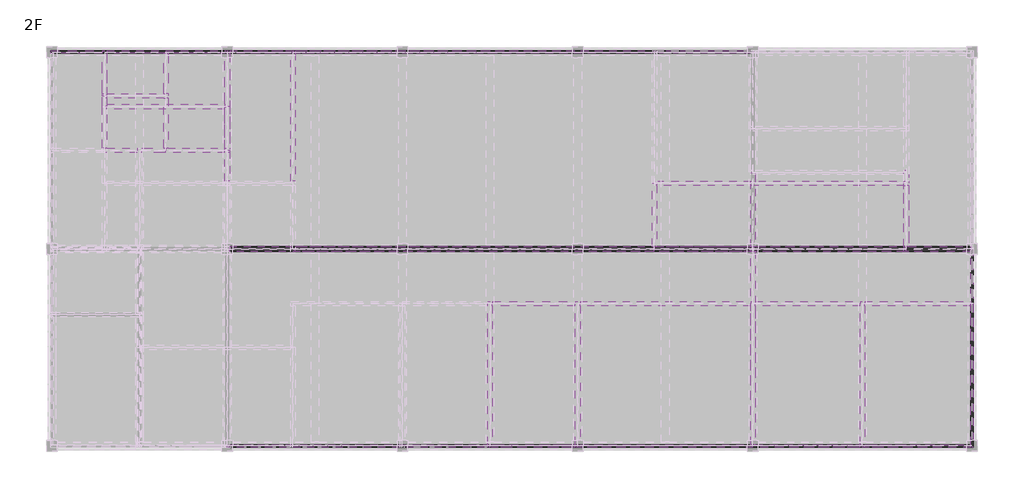
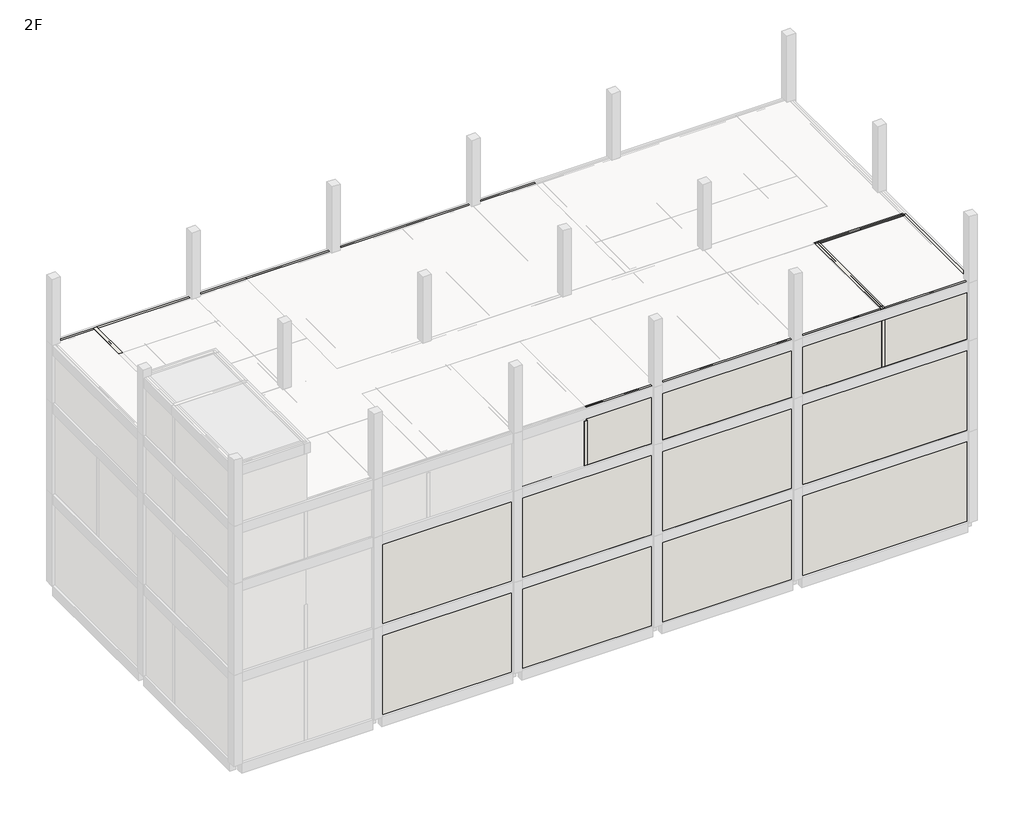
# One storey, part 2 of 7: 54 walls.
"""IFC4 building model written with IfcOpenShell, lengths in millimetres."""

from ifc_helpers import new_model, si_unit, frame, origin, place, context, project, spatial, polyline, outline, extrude, faceted_brep, element, save

model = new_model("IFC4")

# Units and contexts
model_context = context("Model", 3, world=origin())
ifc_project = project(units=[si_unit("LENGTHUNIT", "METRE", prefix="MILLI")], contexts=[model_context])

# Site, building, storey
site = spatial("IfcSite", under=ifc_project)
building = spatial("IfcBuilding", under=site)
storey = spatial("IfcBuildingStorey", under=building, Name="2F", Elevation=3500.0)

# Walls
placement = place(None, origin())
element("IfcWall", 1, ObjectType="WA211_Exterior-Cement Brick-90mm", at=placement, inside=storey, context=model_context, shape_type="Brep", body=[
    faceted_brep([(45402.6521483, 181866.8614395, 3500.0), (45516.6521483, 181866.8614395, 3500.0), (77352.6521483, 181866.8614395, 3500.0), (77352.6521483, 181866.8614395, 9000.0), (45516.6521483, 181866.8614395, 9000.0), (45402.6521483, 181866.8614395, 9000.0), (45402.6521483, 181980.8614395, 3500.0), (45402.6521483, 181980.8614395, 9000.0), (77352.6521483, 181980.8614395, 9000.0), (77352.6521483, 181980.8614395, 3500.0)], [[[0, 1, 2, 3, 4, 5]], [[6, 7, 8, 9]], [[2, 1, 0, 6, 9]], [[5, 4, 3, 8, 7]], [[0, 5, 7, 6]], [[3, 2, 9, 8]]]),
])
element("IfcWall", 2, ObjectType="WA211_Exterior-Cement Brick-90mm", at=placement, inside=storey, context=model_context, shape_type="SweptSolid", body=[
    extrude(outline(polyline([(53566.6521483, 163980.8614395), (87402.6521483, 163980.8614395), (87402.6521483, 163866.8614395), (53566.6521483, 163866.8614395), (53566.6521483, 163980.8614395)])), frame((0.0, 0.0, 3500.0), z_axis=(0.0, 0.0, 1.0), x_axis=(1.0, 0.0, 0.0)), (0.0, 0.0, 1.0), 5500.0),
])
element("IfcWall", 3, ObjectType="WA211_Exterior-Cement Brick-90mm", at=placement, inside=storey, context=model_context, shape_type="Brep", body=[
    faceted_brep([(87402.6521483, 172923.8614395, 3500.0), (87402.6521483, 172816.8614395, 3500.0), (87402.6521483, 163980.8614395, 3500.0), (87402.6521483, 163866.8614395, 3500.0), (87402.6521483, 163866.8614395, 9000.0), (87402.6521483, 163980.8614395, 9000.0), (87402.6521483, 172816.8614395, 9000.0), (87402.6521483, 172923.8614395, 9000.0), (87516.6521483, 172923.8614395, 3500.0), (87516.6521483, 172923.8614395, 9000.0), (87516.6521483, 163866.8614395, 9000.0), (87516.6521483, 163866.8614395, 3500.0)], [[[0, 1, 2, 3, 4, 5, 6, 7]], [[8, 9, 10, 11]], [[3, 2, 1, 0, 8, 11]], [[7, 6, 5, 4, 10, 9]], [[0, 7, 9, 8]], [[4, 3, 11, 10]]]),
])
element("IfcWall", 4, ObjectType="WA211_Exterior-Cement Brick-90mm", at=placement, inside=storey, context=model_context, shape_type="SweptSolid", body=[
    extrude(outline(polyline([(9000.0, 53566.6521483), (9000.0, 77352.6521483), (12400.0, 77352.6521483), (12400.0, 77459.6521483), (14500.0, 77459.6521483), (14500.0, 53459.6521483), (12400.0, 53459.6521483), (12400.0, 53566.6521483), (9000.0, 53566.6521483)])), frame((0.0, 181866.8614395, 0.0), z_axis=(0.0, 1.0, 0.0), x_axis=(0.0, 0.0, 1.0)), (0.0, 0.0, 1.0), 114.0),
])
element("IfcWall", 5, ObjectType="WA211_Exterior-Cement Brick-90mm", at=placement, inside=storey, context=model_context, shape_type="Brep", body=[
    faceted_brep([(77459.6521483, 163980.8614395, 9000.0), (77352.6521483, 163980.8614395, 9000.0), (53566.6521483, 163980.8614395, 9000.0), (53566.6521483, 163980.8614395, 12000.0), (53459.6521483, 163980.8614395, 12000.0), (53459.6521483, 163980.8614395, 14500.0), (77352.6521483, 163980.8614395, 14500.0), (77459.6521483, 163980.8614395, 14500.0), (77459.6521483, 163866.8614395, 9000.0), (77459.6521483, 163866.8614395, 14500.0), (53459.6521483, 163866.8614395, 14500.0), (53459.6521483, 163866.8614395, 12000.0), (53566.6521483, 163866.8614395, 12000.0), (53566.6521483, 163866.8614395, 9000.0)], [[[0, 1, 2, 3, 4, 5, 6, 7]], [[8, 9, 10, 11, 12, 13]], [[2, 1, 0, 8, 13]], [[7, 6, 5, 10, 9]], [[0, 7, 9, 8]], [[5, 4, 11, 10]], [[11, 4, 3, 12]], [[3, 2, 13, 12]]]),
])
element("IfcWall", 6, ObjectType="WA211_Exterior-Cement Brick-90mm", at=placement, inside=storey, context=model_context, shape_type="Brep", body=[
    faceted_brep([(87402.6521483, 163980.8614395, 9000.0), (77566.6521483, 163980.8614395, 9000.0), (77459.6521483, 163980.8614395, 9000.0), (77459.6521483, 163980.8614395, 14500.0), (77566.6521483, 163980.8614395, 14500.0), (87402.6521483, 163980.8614395, 14500.0), (87402.6521483, 163866.8614395, 9000.0), (87402.6521483, 163866.8614395, 14500.0), (77459.6521483, 163866.8614395, 14500.0), (77459.6521483, 163866.8614395, 9000.0)], [[[0, 1, 2, 3, 4, 5]], [[6, 7, 8, 9]], [[2, 1, 0, 6, 9]], [[3, 2, 9, 8]], [[5, 4, 3, 8, 7]], [[0, 5, 7, 6]]]),
])
element("IfcWall", 7, ObjectType="WA211_Exterior-Cement Brick-90mm", at=placement, inside=storey, context=model_context, shape_type="Brep", body=[
    faceted_brep([(87402.6521483, 172923.8614395, 9000.0), (87402.6521483, 172816.8614395, 9000.0), (87402.6521483, 163980.8614395, 9000.0), (87402.6521483, 163866.8614395, 9000.0), (87402.6521483, 163866.8614395, 14500.0), (87402.6521483, 163980.8614395, 14500.0), (87402.6521483, 172816.8614395, 14500.0), (87402.6521483, 172923.8614395, 14500.0), (87516.6521483, 172923.8614395, 9000.0), (87516.6521483, 172923.8614395, 14500.0), (87516.6521483, 163866.8614395, 14500.0), (87516.6521483, 163866.8614395, 9000.0)], [[[0, 1, 2, 3, 4, 5, 6, 7]], [[8, 9, 10, 11]], [[3, 2, 1, 0, 8, 11]], [[7, 6, 5, 4, 10, 9]], [[0, 7, 9, 8]], [[4, 3, 11, 10]]]),
])
element("IfcWall", 8, ObjectType="WA211_Exterior-Cement Brick-90mm", at=placement, inside=storey, context=model_context, shape_type="Brep", body=[
    faceted_brep([(45402.6521483, 181866.8614395, 9000.0), (45516.6521483, 181866.8614395, 9000.0), (47752.6521483, 181866.8614395, 9000.0), (47752.6521483, 181866.8614395, 14500.0), (45516.6521483, 181866.8614395, 14500.0), (45402.6521483, 181866.8614395, 14500.0), (45402.6521483, 181980.8614395, 9000.0), (45402.6521483, 181980.8614395, 14500.0), (47752.6521483, 181980.8614395, 14500.0), (47752.6521483, 181980.8614395, 9000.0)], [[[0, 1, 2, 3, 4, 5]], [[6, 7, 8, 9]], [[2, 1, 0, 6, 9]], [[5, 4, 3, 8, 7]], [[0, 5, 7, 6]], [[3, 2, 9, 8]]]),
])
element("IfcWall", 9, ObjectType="WA211_Exterior-Cement Brick-90mm", at=placement, inside=storey, context=model_context, shape_type="Brep", body=[
    faceted_brep([(50659.6521483, 181866.8614395, 14500.0), (50659.6521483, 181866.8614395, 9000.0), (50766.6521483, 181866.8614395, 9000.0), (53352.6521483, 181866.8614395, 9000.0), (53352.6521483, 181866.8614395, 12400.0), (53459.6521483, 181866.8614395, 12400.0), (53459.6521483, 181866.8614395, 14500.0), (50659.6521483, 181980.8614395, 9000.0), (50659.6521483, 181980.8614395, 14500.0), (53459.6521483, 181980.8614395, 14500.0), (53459.6521483, 181980.8614395, 12400.0), (53352.6521483, 181980.8614395, 12400.0), (53352.6521483, 181980.8614395, 9000.0)], [[[0, 1, 2, 3, 4, 5, 6]], [[7, 8, 9, 10, 11, 12]], [[3, 2, 1, 7, 12]], [[0, 6, 9, 8]], [[6, 5, 10, 9]], [[10, 5, 4, 11]], [[4, 3, 12, 11]], [[0, 8, 7, 1]]]),
])
element("IfcWall", 10, ObjectType="WA211_Exterior-Cement Brick-90mm", at=placement, inside=storey, context=model_context, shape_type="Brep", body=[
    faceted_brep([(47966.6521483, 181866.8614395, 9000.0), (50552.6521483, 181866.8614395, 9000.0), (50659.6521483, 181866.8614395, 9000.0), (50659.6521483, 181866.8614395, 14500.0), (47966.6521483, 181866.8614395, 14500.0), (47966.6521483, 181980.8614395, 9000.0), (47966.6521483, 181980.8614395, 14500.0), (50659.6521483, 181980.8614395, 14500.0), (50659.6521483, 181980.8614395, 9000.0)], [[[0, 1, 2, 3, 4]], [[5, 6, 7, 8]], [[2, 1, 0, 5, 8]], [[4, 3, 7, 6]], [[0, 4, 6, 5]], [[2, 8, 7, 3]]]),
])
element("IfcWall", 11, ObjectType="WA211_Exterior-Cement Brick-90mm", at=placement, inside=storey, context=model_context, shape_type="SweptSolid", body=[
    extrude(outline(polyline([(14500.0, 69352.6521483), (17200.0, 69352.6521483), (17200.0, 69459.6521483), (18000.0, 69459.6521483), (18000.0, 65459.6521483), (17200.0, 65459.6521483), (17200.0, 65566.6521483), (14500.0, 65566.6521483), (14500.0, 69352.6521483)])), frame((0.0, 163866.8614395, 0.0), z_axis=(0.0, 1.0, 0.0), x_axis=(0.0, 0.0, 1.0)), (0.0, 0.0, 1.0), 114.0),
])
element("IfcWall", 12, ObjectType="WA211_Exterior-Cement Brick-90mm", at=placement, inside=storey, context=model_context, shape_type="Brep", body=[
    faceted_brep([(77459.6521483, 163980.8614395, 18000.0), (77459.6521483, 163980.8614395, 14500.0), (77352.6521483, 163980.8614395, 14500.0), (69566.6521483, 163980.8614395, 14500.0), (69566.6521483, 163980.8614395, 17200.0), (69459.6521483, 163980.8614395, 17200.0), (69459.6521483, 163980.8614395, 18000.0), (77459.6521483, 163866.8614395, 14500.0), (77459.6521483, 163866.8614395, 18000.0), (69459.6521483, 163866.8614395, 18000.0), (69459.6521483, 163866.8614395, 17200.0), (69566.6521483, 163866.8614395, 17200.0), (69566.6521483, 163866.8614395, 14500.0)], [[[0, 1, 2, 3, 4, 5, 6]], [[7, 8, 9, 10, 11, 12]], [[3, 2, 1, 7, 12]], [[0, 6, 9, 8]], [[6, 5, 10, 9]], [[10, 5, 4, 11]], [[4, 3, 12, 11]], [[0, 8, 7, 1]]]),
])
element("IfcWall", 13, ObjectType="WA211_Exterior-Cement Brick-90mm", at=placement, inside=storey, context=model_context, shape_type="SweptSolid", body=[
    extrude(outline(polyline([(14500.0, 56566.6521483), (14500.0, 72852.6521483), (17200.0, 72852.6521483), (17200.0, 72959.6521483), (18000.0, 72959.6521483), (18000.0, 56459.6521483), (17200.0, 56459.6521483), (17200.0, 56566.6521483), (14500.0, 56566.6521483)])), frame((0.0, 181866.8614395, 0.0), z_axis=(0.0, 1.0, 0.0), x_axis=(0.0, 0.0, 1.0)), (0.0, 0.0, 1.0), 114.0),
])
element("IfcWall", 14, ObjectType="WA211_Exterior-Cement Brick-90mm", at=placement, inside=storey, context=model_context, shape_type="Brep", body=[
    faceted_brep([(82352.6521483, 163980.8614395, 14500.0), (77566.6521483, 163980.8614395, 14500.0), (77459.6521483, 163980.8614395, 14500.0), (77459.6521483, 163980.8614395, 18000.0), (82352.6521483, 163980.8614395, 18000.0), (82352.6521483, 163866.8614395, 14500.0), (82352.6521483, 163866.8614395, 18000.0), (77459.6521483, 163866.8614395, 18000.0), (77459.6521483, 163866.8614395, 14500.0)], [[[0, 1, 2, 3, 4]], [[5, 6, 7, 8]], [[2, 1, 0, 5, 8]], [[4, 3, 7, 6]], [[2, 8, 7, 3]], [[0, 4, 6, 5]]]),
])
element("IfcWall", 15, ObjectType="WA211_Exterior-Cement Brick-90mm", at=placement, inside=storey, context=model_context, shape_type="SweptSolid", body=[
    extrude(outline(polyline([(82566.6521483, 163980.8614395), (87402.6521483, 163980.8614395), (87402.6521483, 163866.8614395), (82566.6521483, 163866.8614395), (82566.6521483, 163980.8614395)])), frame((0.0, 0.0, 14500.0), z_axis=(0.0, 0.0, 1.0), x_axis=(1.0, 0.0, 0.0)), (0.0, 0.0, 1.0), 3500.0),
])
element("IfcWall", 16, ObjectType="WA211_Exterior-Cement Brick-90mm", at=placement, inside=storey, context=model_context, shape_type="Brep", body=[
    faceted_brep([(87402.6521483, 170423.8614395, 14500.0), (87402.6521483, 170316.8614395, 14500.0), (87402.6521483, 163980.8614395, 14500.0), (87402.6521483, 163866.8614395, 14500.0), (87402.6521483, 163866.8614395, 18000.0), (87402.6521483, 163980.8614395, 18000.0), (87402.6521483, 170316.8614395, 18000.0), (87402.6521483, 170423.8614395, 18000.0), (87516.6521483, 170423.8614395, 14500.0), (87516.6521483, 170423.8614395, 18000.0), (87516.6521483, 163866.8614395, 18000.0), (87516.6521483, 163866.8614395, 14500.0)], [[[0, 1, 2, 3, 4, 5, 6, 7]], [[8, 9, 10, 11]], [[3, 2, 1, 0, 8, 11]], [[7, 6, 5, 4, 10, 9]], [[0, 7, 9, 8]], [[4, 3, 11, 10]]]),
])
element("IfcWall", 17, ObjectType="WA211_Exterior-Cement Brick-90mm", at=placement, inside=storey, context=model_context, shape_type="SweptSolid", body=[
    extrude(outline(polyline([(14500.0, 47966.6521483), (14500.0, 53352.6521483), (17200.0, 53352.6521483), (17200.0, 53459.6521483), (18000.0, 53459.6521483), (18000.0, 47966.6521483), (14500.0, 47966.6521483)])), frame((0.0, 181866.8614395, 0.0), z_axis=(0.0, 1.0, 0.0), x_axis=(0.0, 0.0, 1.0)), (0.0, 0.0, 1.0), 114.0),
])
element("IfcWall", 18, ObjectType="WA211_Exterior-Cement Brick-90mm", at=placement, inside=storey, context=model_context, shape_type="SweptSolid", body=[
    extrude(outline(polyline([(14500.0, 53566.6521483), (14500.0, 56352.6521483), (17200.0, 56352.6521483), (17200.0, 56459.6521483), (18000.0, 56459.6521483), (18000.0, 53459.6521483), (17200.0, 53459.6521483), (17200.0, 53566.6521483), (14500.0, 53566.6521483)])), frame((0.0, 181866.8614395, 0.0), z_axis=(0.0, 1.0, 0.0), x_axis=(0.0, 0.0, 1.0)), (0.0, 0.0, 1.0), 114.0),
])
element("IfcWall", 19, ObjectType="WA211_Exterior-Cement Brick-90mm", at=placement, inside=storey, context=model_context, shape_type="Brep", body=[
    faceted_brep([(45402.6521483, 181866.8614395, 14500.0), (45516.6521483, 181866.8614395, 14500.0), (47752.6521483, 181866.8614395, 14500.0), (47752.6521483, 181866.8614395, 18000.0), (45516.6521483, 181866.8614395, 18000.0), (45402.6521483, 181866.8614395, 18000.0), (45402.6521483, 181980.8614395, 14500.0), (45402.6521483, 181980.8614395, 18000.0), (47752.6521483, 181980.8614395, 18000.0), (47752.6521483, 181980.8614395, 14500.0)], [[[0, 1, 2, 3, 4, 5]], [[6, 7, 8, 9]], [[2, 1, 0, 6, 9]], [[5, 4, 3, 8, 7]], [[3, 2, 9, 8]], [[0, 5, 7, 6]]]),
])
element("IfcWall", 20, ObjectType="WA221_Interior-Cement Block-190mm", at=placement, inside=storey, context=model_context, shape_type="SweptSolid", body=[
    extrude(outline(polyline([(53566.6521483, 173030.8614395), (77352.6521483, 173030.8614395), (77352.6521483, 172816.8614395), (53566.6521483, 172816.8614395), (53566.6521483, 173030.8614395)])), frame((0.0, 0.0, 3500.0), z_axis=(0.0, 0.0, 1.0), x_axis=(1.0, 0.0, 0.0)), (0.0, 0.0, 1.0), 5500.0),
])
element("IfcWall", 21, ObjectType="WA221_Interior-Cement Block-190mm", at=placement, inside=storey, context=model_context, shape_type="Brep", body=[
    faceted_brep([(77566.6521483, 172816.8614395, 3500.0), (87402.6521483, 172816.8614395, 3500.0), (87402.6521483, 172816.8614395, 9000.0), (77566.6521483, 172816.8614395, 9000.0), (77566.6521483, 173030.8614395, 3500.0), (77566.6521483, 173030.8614395, 9000.0), (87402.6521483, 173030.8614395, 9000.0), (87402.6521483, 173030.8614395, 3500.0), (87402.6521483, 172923.8614395, 3500.0), (87402.6521483, 172923.8614395, 9000.0)], [[[0, 1, 2, 3]], [[4, 5, 6, 7]], [[1, 0, 4, 7, 8]], [[3, 2, 9, 6, 5]], [[0, 3, 5, 4]], [[2, 1, 8, 7, 6, 9]]]),
])
element("IfcWall", 22, ObjectType="WA221_Interior-Cement Block-190mm", at=placement, inside=storey, context=model_context, shape_type="Brep", body=[
    faceted_brep([(77459.6521483, 173030.8614395, 9000.0), (77352.6521483, 173030.8614395, 9000.0), (53566.6521483, 173030.8614395, 9000.0), (53566.6521483, 173030.8614395, 12400.0), (77352.6521483, 173030.8614395, 12400.0), (77459.6521483, 173030.8614395, 12400.0), (77459.6521483, 172816.8614395, 9000.0), (77459.6521483, 172816.8614395, 12400.0), (77352.6521483, 172816.8614395, 12400.0), (53566.6521483, 172816.8614395, 12400.0), (53566.6521483, 172816.8614395, 12000.0), (53566.6521483, 172816.8614395, 9000.0), (77352.6521483, 172816.8614395, 9000.0), (53566.6521483, 172923.8614395, 9000.0)], [[[0, 1, 2, 3, 4, 5]], [[6, 7, 8, 9, 10, 11, 12]], [[2, 1, 0, 6, 12, 11, 13]], [[5, 4, 3, 9, 8, 7]], [[0, 5, 7, 6]], [[2, 13, 11, 10, 9, 3]]]),
])
element("IfcWall", 23, ObjectType="WA221_Interior-Cement Block-190mm", at=placement, inside=storey, context=model_context, shape_type="Brep", body=[
    faceted_brep([(77352.6521483, 176316.8614395, 9000.0), (77352.6521483, 173030.8614395, 9000.0), (77352.6521483, 173030.8614395, 12400.0), (77352.6521483, 176423.8614395, 12400.0), (77352.6521483, 176423.8614395, 11700.0), (77352.6521483, 176316.8614395, 11700.0), (77566.6521483, 176316.8614395, 9000.0), (77566.6521483, 176316.8614395, 11700.0), (77566.6521483, 176423.8614395, 11700.0), (77566.6521483, 176423.8614395, 12400.0), (77566.6521483, 173030.8614395, 12400.0), (77566.6521483, 173030.8614395, 9000.0), (77459.6521483, 173030.8614395, 9000.0), (77459.6521483, 173030.8614395, 12400.0)], [[[0, 1, 2, 3, 4, 5]], [[6, 7, 8, 9, 10, 11]], [[1, 0, 6, 11, 12]], [[3, 2, 13, 10, 9]], [[2, 1, 12, 11, 10, 13]], [[4, 3, 9, 8]], [[4, 8, 7, 5]], [[0, 5, 7, 6]]]),
])
element("IfcWall", 24, ObjectType="WA221_Interior-Cement Block-190mm", at=placement, inside=storey, context=model_context, shape_type="Brep", body=[
    faceted_brep([(53566.6521483, 177530.8614395, 9000.0), (53566.6521483, 181866.8614395, 9000.0), (53566.6521483, 181980.8614395, 9000.0), (53566.6521483, 181980.8614395, 12400.0), (53566.6521483, 181866.8614395, 12400.0), (53566.6521483, 177423.8614395, 12400.0), (53566.6521483, 177423.8614395, 11700.0), (53566.6521483, 177530.8614395, 11700.0), (53352.6521483, 177530.8614395, 9000.0), (53352.6521483, 177530.8614395, 11700.0), (53352.6521483, 177423.8614395, 11700.0), (53352.6521483, 177423.8614395, 12400.0), (53352.6521483, 181866.8614395, 12400.0), (53352.6521483, 181980.8614395, 12400.0), (53352.6521483, 181980.8614395, 9000.0), (53352.6521483, 181866.8614395, 9000.0), (53459.6521483, 181980.8614395, 12400.0)], [[[0, 1, 2, 3, 4, 5, 6, 7]], [[8, 9, 10, 11, 12, 13, 14, 15]], [[2, 1, 0, 8, 15, 14]], [[5, 4, 3, 16, 13, 12, 11]], [[3, 2, 14, 13, 16]], [[6, 5, 11, 10]], [[6, 10, 9, 7]], [[0, 7, 9, 8]]]),
])
element("IfcWall", 25, ObjectType="WA221_Interior-Cement Block-190mm", at=placement, inside=storey, context=model_context, shape_type="Brep", body=[
    faceted_brep([(77566.6521483, 163980.8614395, 9000.0), (77566.6521483, 172816.8614395, 9000.0), (77566.6521483, 172816.8614395, 14500.0), (77566.6521483, 163980.8614395, 14500.0), (77352.6521483, 163980.8614395, 9000.0), (77352.6521483, 163980.8614395, 14500.0), (77352.6521483, 172816.8614395, 14500.0), (77352.6521483, 172816.8614395, 12400.0), (77352.6521483, 172816.8614395, 9000.0), (77459.6521483, 163980.8614395, 9000.0), (77459.6521483, 172816.8614395, 9000.0), (77459.6521483, 163980.8614395, 14500.0)], [[[0, 1, 2, 3]], [[4, 5, 6, 7, 8]], [[1, 0, 9, 4, 8, 10]], [[3, 2, 6, 5, 11]], [[1, 10, 8, 7, 6, 2]], [[0, 3, 11, 5, 4, 9]]]),
])
element("IfcWall", 26, ObjectType="WA221_Interior-Cement Block-190mm", at=placement, inside=storey, context=model_context, shape_type="Brep", body=[
    faceted_brep([(77459.6521483, 172816.8614395, 9000.0), (77566.6521483, 172816.8614395, 9000.0), (84459.6521483, 172816.8614395, 9000.0), (84459.6521483, 172816.8614395, 14500.0), (77566.6521483, 172816.8614395, 14500.0), (77352.6521483, 172816.8614395, 14500.0), (77352.6521483, 172816.8614395, 12400.0), (77459.6521483, 172816.8614395, 12400.0), (77459.6521483, 173030.8614395, 9000.0), (77459.6521483, 173030.8614395, 12400.0), (77352.6521483, 173030.8614395, 12400.0), (77352.6521483, 173030.8614395, 14500.0), (84459.6521483, 173030.8614395, 14500.0), (84459.6521483, 173030.8614395, 9000.0), (84352.6521483, 173030.8614395, 9000.0), (77566.6521483, 173030.8614395, 9000.0)], [[[0, 1, 2, 3, 4, 5, 6, 7]], [[8, 9, 10, 11, 12, 13, 14, 15]], [[2, 1, 0, 8, 15, 14, 13]], [[5, 4, 3, 12, 11]], [[0, 7, 9, 8]], [[6, 10, 9, 7]], [[6, 5, 11, 10]], [[2, 13, 12, 3]]]),
])
element("IfcWall", 27, ObjectType="WA221_Interior-Cement Block-190mm", at=placement, inside=storey, context=model_context, shape_type="Brep", body=[
    faceted_brep([(84459.6521483, 172816.8614395, 14500.0), (84459.6521483, 172816.8614395, 9000.0), (87402.6521483, 172816.8614395, 9000.0), (87402.6521483, 172816.8614395, 14500.0), (84459.6521483, 173030.8614395, 9000.0), (84459.6521483, 173030.8614395, 14500.0), (87402.6521483, 173030.8614395, 14500.0), (87402.6521483, 173030.8614395, 9000.0), (84566.6521483, 173030.8614395, 9000.0), (87402.6521483, 172923.8614395, 9000.0), (87402.6521483, 172923.8614395, 14500.0)], [[[0, 1, 2, 3]], [[4, 5, 6, 7, 8]], [[2, 1, 4, 8, 7, 9]], [[0, 3, 10, 6, 5]], [[3, 2, 9, 7, 6, 10]], [[0, 5, 4, 1]]]),
])
element("IfcWall", 28, ObjectType="WA221_Interior-Cement Block-190mm", at=placement, inside=storey, context=model_context, shape_type="Brep", body=[
    faceted_brep([(84352.6521483, 176530.8614395, 9000.0), (84352.6521483, 176316.8614395, 9000.0), (84352.6521483, 173030.8614395, 9000.0), (84352.6521483, 173030.8614395, 11700.0), (84352.6521483, 176316.8614395, 11700.0), (84352.6521483, 176530.8614395, 11700.0), (84566.6521483, 176530.8614395, 9000.0), (84566.6521483, 176530.8614395, 11700.0), (84566.6521483, 173030.8614395, 11700.0), (84566.6521483, 173030.8614395, 9000.0), (84459.6521483, 173030.8614395, 9000.0)], [[[0, 1, 2, 3, 4, 5]], [[6, 7, 8, 9]], [[2, 1, 0, 6, 9, 10]], [[5, 4, 3, 8, 7]], [[0, 5, 7, 6]], [[3, 2, 10, 9, 8]]]),
])
element("IfcWall", 29, ObjectType="WA221_Interior-Cement Block-190mm", at=placement, inside=storey, context=model_context, shape_type="Brep", body=[
    faceted_brep([(47752.6521483, 181980.8614395, 9000.0), (47752.6521483, 181866.8614395, 9000.0), (47752.6521483, 180030.8614395, 9000.0), (47752.6521483, 180030.8614395, 11700.0), (47752.6521483, 179923.8614395, 11700.0), (47752.6521483, 179923.8614395, 14500.0), (47752.6521483, 181866.8614395, 14500.0), (47752.6521483, 181980.8614395, 14500.0), (47966.6521483, 181980.8614395, 9000.0), (47966.6521483, 181980.8614395, 14500.0), (47966.6521483, 181866.8614395, 14500.0), (47966.6521483, 179923.8614395, 14500.0), (47966.6521483, 179923.8614395, 11700.0), (47966.6521483, 180030.8614395, 11700.0), (47966.6521483, 180030.8614395, 9000.0), (47966.6521483, 181866.8614395, 9000.0)], [[[0, 1, 2, 3, 4, 5, 6, 7]], [[8, 9, 10, 11, 12, 13, 14, 15]], [[2, 1, 0, 8, 15, 14]], [[7, 6, 5, 11, 10, 9]], [[0, 7, 9, 8]], [[5, 4, 12, 11]], [[12, 4, 3, 13]], [[3, 2, 14, 13]]]),
])
element("IfcWall", 30, ObjectType="WA221_Interior-Cement Block-190mm", at=placement, inside=storey, context=model_context, shape_type="Brep", body=[
    faceted_brep([(47752.6521483, 179816.8614395, 9000.0), (47752.6521483, 177530.8614395, 9000.0), (47752.6521483, 177530.8614395, 14500.0), (47752.6521483, 179923.8614395, 14500.0), (47752.6521483, 179923.8614395, 11700.0), (47752.6521483, 179816.8614395, 11700.0), (47966.6521483, 179816.8614395, 9000.0), (47966.6521483, 179816.8614395, 11700.0), (47966.6521483, 179923.8614395, 11700.0), (47966.6521483, 179923.8614395, 14500.0), (47966.6521483, 177530.8614395, 14500.0), (47966.6521483, 177530.8614395, 11700.0), (47966.6521483, 177530.8614395, 9000.0), (47859.6521483, 177530.8614395, 9000.0)], [[[0, 1, 2, 3, 4, 5]], [[6, 7, 8, 9, 10, 11, 12]], [[1, 0, 6, 12, 13]], [[3, 2, 10, 9]], [[1, 13, 12, 11, 10, 2]], [[4, 3, 9, 8]], [[4, 8, 7, 5]], [[0, 5, 7, 6]]]),
])
element("IfcWall", 31, ObjectType="WA221_Interior-Cement Block-190mm", at=placement, inside=storey, context=model_context, shape_type="Brep", body=[
    faceted_brep([(49352.6521483, 177530.8614395, 9000.0), (47966.6521483, 177530.8614395, 9000.0), (47859.6521483, 177530.8614395, 9000.0), (47859.6521483, 177530.8614395, 11700.0), (47966.6521483, 177530.8614395, 11700.0), (49352.6521483, 177530.8614395, 11700.0), (49352.6521483, 177316.8614395, 9000.0), (49352.6521483, 177316.8614395, 11700.0), (47966.6521483, 177316.8614395, 11700.0), (47859.6521483, 177316.8614395, 11700.0), (47859.6521483, 177316.8614395, 9000.0)], [[[0, 1, 2, 3, 4, 5]], [[6, 7, 8, 9, 10]], [[2, 1, 0, 6, 10]], [[3, 2, 10, 9]], [[5, 4, 3, 9, 8, 7]], [[0, 5, 7, 6]]]),
])
element("IfcWall", 32, ObjectType="WA221_Interior-Cement Block-190mm", at=placement, inside=storey, context=model_context, shape_type="Brep", body=[
    faceted_brep([(50552.6521483, 181866.8614395, 9000.0), (50552.6521483, 180030.8614395, 9000.0), (50552.6521483, 180030.8614395, 11700.0), (50552.6521483, 181866.8614395, 11700.0), (50766.6521483, 181866.8614395, 9000.0), (50766.6521483, 181866.8614395, 11700.0), (50766.6521483, 180030.8614395, 11700.0), (50766.6521483, 180030.8614395, 9000.0), (50659.6521483, 181866.8614395, 9000.0)], [[[0, 1, 2, 3]], [[4, 5, 6, 7]], [[1, 0, 8, 4, 7]], [[3, 2, 6, 5]], [[0, 3, 5, 4, 8]], [[2, 1, 7, 6]]]),
])
element("IfcWall", 33, ObjectType="WA221_Interior-Cement Block-190mm", at=placement, inside=storey, context=model_context, shape_type="Brep", body=[
    faceted_brep([(50766.6521483, 177530.8614395, 9000.0), (50766.6521483, 179816.8614395, 9000.0), (50766.6521483, 179816.8614395, 11700.0), (50766.6521483, 177530.8614395, 11700.0), (50552.6521483, 177530.8614395, 9000.0), (50552.6521483, 177530.8614395, 11700.0), (50552.6521483, 179816.8614395, 11700.0), (50552.6521483, 179816.8614395, 9000.0), (50659.6521483, 177530.8614395, 9000.0), (50659.6521483, 177530.8614395, 11700.0)], [[[0, 1, 2, 3]], [[4, 5, 6, 7]], [[1, 0, 8, 4, 7]], [[3, 2, 6, 5, 9]], [[0, 3, 9, 5, 4, 8]], [[2, 1, 7, 6]]]),
])
element("IfcWall", 34, ObjectType="WA221_Interior-Cement Block-190mm", at=placement, inside=storey, context=model_context, shape_type="Brep", body=[
    faceted_brep([(50659.6521483, 177316.8614395, 9000.0), (53352.6521483, 177316.8614395, 9000.0), (53566.6521483, 177316.8614395, 9000.0), (53566.6521483, 177316.8614395, 11700.0), (53352.6521483, 177316.8614395, 11700.0), (50659.6521483, 177316.8614395, 11700.0), (50659.6521483, 177530.8614395, 9000.0), (50659.6521483, 177530.8614395, 11700.0), (50766.6521483, 177530.8614395, 11700.0), (53352.6521483, 177530.8614395, 11700.0), (53566.6521483, 177530.8614395, 11700.0), (53566.6521483, 177530.8614395, 9000.0), (53352.6521483, 177530.8614395, 9000.0), (50766.6521483, 177530.8614395, 9000.0), (53566.6521483, 177423.8614395, 11700.0)], [[[0, 1, 2, 3, 4, 5]], [[6, 7, 8, 9, 10, 11, 12, 13]], [[2, 1, 0, 6, 13, 12, 11]], [[5, 4, 3, 14, 10, 9, 8, 7]], [[0, 5, 7, 6]], [[3, 2, 11, 10, 14]]]),
])
element("IfcWall", 35, ObjectType="WA221_Interior-Cement Block-190mm", at=placement, inside=storey, context=model_context, shape_type="Brep", body=[
    faceted_brep([(50766.6521483, 180030.8614395, 9000.0), (50552.6521483, 180030.8614395, 9000.0), (47966.6521483, 180030.8614395, 9000.0), (47752.6521483, 180030.8614395, 9000.0), (47752.6521483, 180030.8614395, 11700.0), (47966.6521483, 180030.8614395, 11700.0), (50552.6521483, 180030.8614395, 11700.0), (50766.6521483, 180030.8614395, 11700.0), (50766.6521483, 179816.8614395, 9000.0), (50766.6521483, 179816.8614395, 11700.0), (50552.6521483, 179816.8614395, 11700.0), (47966.6521483, 179816.8614395, 11700.0), (47752.6521483, 179816.8614395, 11700.0), (47752.6521483, 179816.8614395, 9000.0), (47966.6521483, 179816.8614395, 9000.0), (50552.6521483, 179816.8614395, 9000.0), (47752.6521483, 179923.8614395, 11700.0)], [[[0, 1, 2, 3, 4, 5, 6, 7]], [[8, 9, 10, 11, 12, 13, 14, 15]], [[3, 2, 1, 0, 8, 15, 14, 13]], [[7, 6, 5, 4, 16, 12, 11, 10, 9]], [[0, 7, 9, 8]], [[4, 3, 13, 12, 16]]]),
])
element("IfcWall", 36, ObjectType="WA221_Interior-Cement Block-190mm", at=placement, inside=storey, context=model_context, shape_type="Brep", body=[
    faceted_brep([(50659.6521483, 177530.8614395, 9000.0), (50552.6521483, 177530.8614395, 9000.0), (49566.6521483, 177530.8614395, 9000.0), (49566.6521483, 177530.8614395, 11700.0), (50552.6521483, 177530.8614395, 11700.0), (50659.6521483, 177530.8614395, 11700.0), (50659.6521483, 177316.8614395, 9000.0), (50659.6521483, 177316.8614395, 11700.0), (49566.6521483, 177316.8614395, 11700.0), (49566.6521483, 177316.8614395, 9000.0)], [[[0, 1, 2, 3, 4, 5]], [[6, 7, 8, 9]], [[2, 1, 0, 6, 9]], [[5, 4, 3, 8, 7]], [[0, 5, 7, 6]], [[3, 2, 9, 8]]]),
])
element("IfcWall", 37, ObjectType="WA221_Interior-Cement Block-190mm", at=placement, inside=storey, context=model_context, shape_type="Brep", body=[
    faceted_brep([(65352.6521483, 170530.8614395, 14500.0), (65352.6521483, 170316.8614395, 14500.0), (65352.6521483, 163980.8614395, 14500.0), (65352.6521483, 163866.8614395, 14500.0), (65352.6521483, 163866.8614395, 17200.0), (65352.6521483, 163980.8614395, 17200.0), (65352.6521483, 170316.8614395, 17200.0), (65352.6521483, 170530.8614395, 17200.0), (65566.6521483, 170530.8614395, 14500.0), (65566.6521483, 170530.8614395, 17200.0), (65566.6521483, 170316.8614395, 17200.0), (65566.6521483, 163980.8614395, 17200.0), (65566.6521483, 163866.8614395, 17200.0), (65566.6521483, 163866.8614395, 14500.0), (65566.6521483, 163980.8614395, 14500.0), (65566.6521483, 170316.8614395, 14500.0), (65459.6521483, 163866.8614395, 17200.0)], [[[0, 1, 2, 3, 4, 5, 6, 7]], [[8, 9, 10, 11, 12, 13, 14, 15]], [[3, 2, 1, 0, 8, 15, 14, 13]], [[7, 6, 5, 4, 16, 12, 11, 10, 9]], [[4, 3, 13, 12, 16]], [[0, 7, 9, 8]]]),
])
element("IfcWall", 38, ObjectType="WA221_Interior-Cement Block-190mm", at=placement, inside=storey, context=model_context, shape_type="Brep", body=[
    faceted_brep([(69566.6521483, 163866.8614395, 14500.0), (69566.6521483, 163980.8614395, 14500.0), (69566.6521483, 170316.8614395, 14500.0), (69566.6521483, 170530.8614395, 14500.0), (69566.6521483, 170530.8614395, 17200.0), (69566.6521483, 170316.8614395, 17200.0), (69566.6521483, 163980.8614395, 17200.0), (69566.6521483, 163866.8614395, 17200.0), (69352.6521483, 163866.8614395, 14500.0), (69352.6521483, 163866.8614395, 17200.0), (69352.6521483, 163980.8614395, 17200.0), (69352.6521483, 170316.8614395, 17200.0), (69352.6521483, 170530.8614395, 17200.0), (69352.6521483, 170530.8614395, 14500.0), (69352.6521483, 170316.8614395, 14500.0), (69352.6521483, 163980.8614395, 14500.0), (69459.6521483, 163866.8614395, 17200.0)], [[[0, 1, 2, 3, 4, 5, 6, 7]], [[8, 9, 10, 11, 12, 13, 14, 15]], [[3, 2, 1, 0, 8, 15, 14, 13]], [[7, 6, 5, 4, 12, 11, 10, 9, 16]], [[4, 3, 13, 12]], [[0, 7, 16, 9, 8]]]),
])
element("IfcWall", 39, ObjectType="WA221_Interior-Cement Block-190mm", at=placement, inside=storey, context=model_context, shape_type="SweptSolid", body=[
    extrude(outline(polyline([(65566.6521483, 170530.8614395), (69352.6521483, 170530.8614395), (69352.6521483, 170316.8614395), (65566.6521483, 170316.8614395), (65566.6521483, 170530.8614395)])), frame((0.0, 0.0, 14500.0), z_axis=(0.0, 0.0, 1.0), x_axis=(1.0, 0.0, 0.0)), (0.0, 0.0, 1.0), 2700.0),
])
element("IfcWall", 40, ObjectType="WA221_Interior-Cement Block-190mm", at=placement, inside=storey, context=model_context, shape_type="Brep", body=[
    faceted_brep([(84566.6521483, 176030.8614395, 14500.0), (84352.6521483, 176030.8614395, 14500.0), (73066.6521483, 176030.8614395, 14500.0), (73066.6521483, 176030.8614395, 17200.0), (84352.6521483, 176030.8614395, 17200.0), (84566.6521483, 176030.8614395, 17200.0), (84566.6521483, 175816.8614395, 14500.0), (84566.6521483, 175816.8614395, 17200.0), (84352.6521483, 175816.8614395, 17200.0), (73066.6521483, 175816.8614395, 17200.0), (73066.6521483, 175816.8614395, 14500.0), (84352.6521483, 175816.8614395, 14500.0), (73066.6521483, 175923.8614395, 14500.0), (73066.6521483, 175923.8614395, 17200.0)], [[[0, 1, 2, 3, 4, 5]], [[6, 7, 8, 9, 10, 11]], [[2, 1, 0, 6, 11, 10, 12]], [[5, 4, 3, 13, 9, 8, 7]], [[0, 5, 7, 6]], [[3, 2, 12, 10, 9, 13]]]),
])
element("IfcWall", 41, ObjectType="WA221_Interior-Cement Block-190mm", at=placement, inside=storey, context=model_context, shape_type="Brep", body=[
    faceted_brep([(77352.6521483, 170530.8614395, 14500.0), (77352.6521483, 170316.8614395, 14500.0), (77352.6521483, 163980.8614395, 14500.0), (77352.6521483, 163980.8614395, 17200.0), (77352.6521483, 170316.8614395, 17200.0), (77352.6521483, 170530.8614395, 17200.0), (77566.6521483, 170530.8614395, 14500.0), (77566.6521483, 170530.8614395, 17200.0), (77566.6521483, 170316.8614395, 17200.0), (77566.6521483, 163980.8614395, 17200.0), (77566.6521483, 163980.8614395, 14500.0), (77566.6521483, 170316.8614395, 14500.0), (77459.6521483, 163980.8614395, 14500.0)], [[[0, 1, 2, 3, 4, 5]], [[6, 7, 8, 9, 10, 11]], [[2, 1, 0, 6, 11, 10, 12]], [[5, 4, 3, 9, 8, 7]], [[0, 5, 7, 6]], [[3, 2, 12, 10, 9]]]),
])
element("IfcWall", 42, ObjectType="WA221_Interior-Cement Block-190mm", at=placement, inside=storey, context=model_context, shape_type="SweptSolid", body=[
    extrude(outline(polyline([(77352.6521483, 170316.8614395), (69566.6521483, 170316.8614395), (69566.6521483, 170530.8614395), (77352.6521483, 170530.8614395), (77352.6521483, 170316.8614395)])), frame((0.0, 0.0, 14500.0), z_axis=(0.0, 0.0, 1.0), x_axis=(1.0, 0.0, 0.0)), (0.0, 0.0, 1.0), 2700.0),
])
element("IfcWall", 43, ObjectType="WA221_Interior-Cement Block-190mm", at=placement, inside=storey, context=model_context, shape_type="Brep", body=[
    faceted_brep([(73066.6521483, 173030.8614395, 14500.0), (73066.6521483, 175816.8614395, 14500.0), (73066.6521483, 175923.8614395, 14500.0), (73066.6521483, 175923.8614395, 17200.0), (73066.6521483, 175816.8614395, 17200.0), (73066.6521483, 173030.8614395, 17200.0), (72852.6521483, 173030.8614395, 14500.0), (72852.6521483, 173030.8614395, 17200.0), (72852.6521483, 175923.8614395, 17200.0), (72852.6521483, 175923.8614395, 14500.0), (72959.6521483, 173030.8614395, 14500.0), (72959.6521483, 173030.8614395, 17200.0)], [[[0, 1, 2, 3, 4, 5]], [[6, 7, 8, 9]], [[2, 1, 0, 10, 6, 9]], [[3, 2, 9, 8]], [[5, 4, 3, 8, 7, 11]], [[0, 5, 11, 7, 6, 10]]]),
])
element("IfcWall", 44, ObjectType="WA221_Interior-Cement Block-190mm", at=placement, inside=storey, context=model_context, shape_type="Brep", body=[
    faceted_brep([(56352.6521483, 181980.8614395, 14500.0), (56352.6521483, 181866.8614395, 14500.0), (56352.6521483, 176030.8614395, 14500.0), (56352.6521483, 176030.8614395, 17200.0), (56352.6521483, 181866.8614395, 17200.0), (56352.6521483, 181980.8614395, 17200.0), (56566.6521483, 181980.8614395, 14500.0), (56566.6521483, 181980.8614395, 17200.0), (56566.6521483, 181866.8614395, 17200.0), (56566.6521483, 176030.8614395, 17200.0), (56566.6521483, 176030.8614395, 14500.0), (56566.6521483, 181866.8614395, 14500.0), (56459.6521483, 181980.8614395, 17200.0)], [[[0, 1, 2, 3, 4, 5]], [[6, 7, 8, 9, 10, 11]], [[2, 1, 0, 6, 11, 10]], [[5, 4, 3, 9, 8, 7, 12]], [[0, 5, 12, 7, 6]], [[3, 2, 10, 9]]]),
])
element("IfcWall", 45, ObjectType="WA221_Interior-Cement Block-190mm", at=placement, inside=storey, context=model_context, shape_type="Brep", body=[
    faceted_brep([(72959.6521483, 173030.8614395, 14500.0), (72852.6521483, 173030.8614395, 14500.0), (56566.6521483, 173030.8614395, 14500.0), (56566.6521483, 173030.8614395, 17200.0), (72852.6521483, 173030.8614395, 17200.0), (72959.6521483, 173030.8614395, 17200.0), (72959.6521483, 172816.8614395, 14500.0), (72959.6521483, 172816.8614395, 17200.0), (56566.6521483, 172816.8614395, 17200.0), (56566.6521483, 172816.8614395, 14500.0)], [[[0, 1, 2, 3, 4, 5]], [[6, 7, 8, 9]], [[2, 1, 0, 6, 9]], [[5, 4, 3, 8, 7]], [[0, 5, 7, 6]], [[3, 2, 9, 8]]]),
])
element("IfcWall", 46, ObjectType="WA221_Interior-Cement Block-190mm", at=placement, inside=storey, context=model_context, shape_type="Brep", body=[
    faceted_brep([(82566.6521483, 163866.8614395, 14500.0), (82566.6521483, 163980.8614395, 14500.0), (82566.6521483, 170316.8614395, 14500.0), (82566.6521483, 170530.8614395, 14500.0), (82566.6521483, 170530.8614395, 18000.0), (82566.6521483, 170316.8614395, 18000.0), (82566.6521483, 163980.8614395, 18000.0), (82566.6521483, 163866.8614395, 18000.0), (82352.6521483, 163866.8614395, 14500.0), (82352.6521483, 163866.8614395, 18000.0), (82352.6521483, 163980.8614395, 18000.0), (82352.6521483, 170530.8614395, 18000.0), (82352.6521483, 170530.8614395, 17200.0), (82352.6521483, 170530.8614395, 14500.0), (82352.6521483, 170316.8614395, 14500.0), (82352.6521483, 163980.8614395, 14500.0)], [[[0, 1, 2, 3, 4, 5, 6, 7]], [[8, 9, 10, 11, 12, 13, 14, 15]], [[3, 2, 1, 0, 8, 15, 14, 13]], [[7, 6, 5, 4, 11, 10, 9]], [[3, 13, 12, 11, 4]], [[0, 7, 9, 8]]]),
])
element("IfcWall", 47, ObjectType="WA221_Interior-Cement Block-190mm", at=placement, inside=storey, context=model_context, shape_type="SweptSolid", body=[
    extrude(outline(polyline([(82352.6521483, 170316.8614395), (77566.6521483, 170316.8614395), (77566.6521483, 170530.8614395), (82352.6521483, 170530.8614395), (82352.6521483, 170316.8614395)])), frame((0.0, 0.0, 14500.0), z_axis=(0.0, 0.0, 1.0), x_axis=(1.0, 0.0, 0.0)), (0.0, 0.0, 1.0), 2700.0),
])
element("IfcWall", 48, ObjectType="WA221_Interior-Cement Block-190mm", at=placement, inside=storey, context=model_context, shape_type="Brep", body=[
    faceted_brep([(82566.6521483, 170316.8614395, 14500.0), (87402.6521483, 170316.8614395, 14500.0), (87402.6521483, 170316.8614395, 18000.0), (82566.6521483, 170316.8614395, 18000.0), (82566.6521483, 170530.8614395, 14500.0), (82566.6521483, 170530.8614395, 18000.0), (87402.6521483, 170530.8614395, 18000.0), (87402.6521483, 170530.8614395, 14500.0), (87402.6521483, 170423.8614395, 14500.0), (87402.6521483, 170423.8614395, 18000.0)], [[[0, 1, 2, 3]], [[4, 5, 6, 7]], [[1, 0, 4, 7, 8]], [[3, 2, 9, 6, 5]], [[0, 3, 5, 4]], [[2, 1, 8, 7, 6, 9]]]),
])
element("IfcWall", 49, ObjectType="WA221_Interior-Cement Block-190mm", at=placement, inside=storey, context=model_context, shape_type="Brep", body=[
    faceted_brep([(84352.6521483, 173030.8614395, 14500.0), (73066.6521483, 173030.8614395, 14500.0), (72959.6521483, 173030.8614395, 14500.0), (72959.6521483, 173030.8614395, 17200.0), (73066.6521483, 173030.8614395, 17200.0), (84352.6521483, 173030.8614395, 17200.0), (84352.6521483, 172816.8614395, 14500.0), (84352.6521483, 172816.8614395, 17200.0), (72959.6521483, 172816.8614395, 17200.0), (72959.6521483, 172816.8614395, 14500.0)], [[[0, 1, 2, 3, 4, 5]], [[6, 7, 8, 9]], [[2, 1, 0, 6, 9]], [[3, 2, 9, 8]], [[5, 4, 3, 8, 7]], [[0, 5, 7, 6]]]),
])
element("IfcWall", 50, ObjectType="WA221_Interior-Cement Block-190mm", at=placement, inside=storey, context=model_context, shape_type="Brep", body=[
    faceted_brep([(84352.6521483, 175816.8614395, 14500.0), (84352.6521483, 173030.8614395, 14500.0), (84352.6521483, 172816.8614395, 14500.0), (84352.6521483, 172816.8614395, 17200.0), (84352.6521483, 173030.8614395, 17200.0), (84352.6521483, 175816.8614395, 17200.0), (84566.6521483, 175816.8614395, 14500.0), (84566.6521483, 175816.8614395, 17200.0), (84566.6521483, 172816.8614395, 17200.0), (84566.6521483, 172816.8614395, 14500.0)], [[[0, 1, 2, 3, 4, 5]], [[6, 7, 8, 9]], [[2, 1, 0, 6, 9]], [[5, 4, 3, 8, 7]], [[0, 5, 7, 6]], [[3, 2, 9, 8]]]),
])
element("IfcWall", 51, ObjectType="WA221_Interior-Cement Block-190mm", at=placement, inside=storey, context=model_context, shape_type="Brep", body=[
    faceted_brep([(53352.6521483, 179530.8614395, 14500.0), (47966.6521483, 179530.8614395, 14500.0), (47966.6521483, 179530.8614395, 17200.0), (53352.6521483, 179530.8614395, 17200.0), (53352.6521483, 179316.8614395, 14500.0), (53352.6521483, 179316.8614395, 17200.0), (47966.6521483, 179316.8614395, 17200.0), (47966.6521483, 179316.8614395, 14500.0), (53352.6521483, 179423.8614395, 14500.0), (47966.6521483, 179423.8614395, 14500.0), (53352.6521483, 179423.8614395, 17200.0)], [[[0, 1, 2, 3]], [[4, 5, 6, 7]], [[1, 0, 8, 4, 7, 9]], [[3, 2, 6, 5, 10]], [[0, 3, 10, 5, 4, 8]], [[2, 1, 9, 7, 6]]]),
])
element("IfcWall", 52, ObjectType="WA221_Interior-Cement Block-190mm", at=placement, inside=storey, context=model_context, shape_type="Brep", body=[
    faceted_brep([(53352.6521483, 179423.8614395, 14500.0), (53352.6521483, 179316.8614395, 14500.0), (53352.6521483, 176030.8614395, 14500.0), (53352.6521483, 176030.8614395, 17200.0), (53352.6521483, 179316.8614395, 17200.0), (53352.6521483, 179423.8614395, 17200.0), (53566.6521483, 179423.8614395, 14500.0), (53566.6521483, 179423.8614395, 17200.0), (53566.6521483, 176030.8614395, 17200.0), (53566.6521483, 176030.8614395, 14500.0), (53459.6521483, 176030.8614395, 14500.0), (53459.6521483, 176030.8614395, 17200.0)], [[[0, 1, 2, 3, 4, 5]], [[6, 7, 8, 9]], [[2, 1, 0, 6, 9, 10]], [[5, 4, 3, 11, 8, 7]], [[0, 5, 7, 6]], [[3, 2, 10, 9, 8, 11]]]),
])
element("IfcWall", 53, ObjectType="WA221_Interior-Cement Block-190mm", at=placement, inside=storey, context=model_context, shape_type="Brep", body=[
    faceted_brep([(53352.6521483, 181980.8614395, 14500.0), (53352.6521483, 181866.8614395, 14500.0), (53352.6521483, 179530.8614395, 14500.0), (53352.6521483, 179423.8614395, 14500.0), (53352.6521483, 179423.8614395, 17200.0), (53352.6521483, 179530.8614395, 17200.0), (53352.6521483, 181866.8614395, 17200.0), (53352.6521483, 181980.8614395, 17200.0), (53566.6521483, 181980.8614395, 14500.0), (53566.6521483, 181980.8614395, 17200.0), (53566.6521483, 181866.8614395, 17200.0), (53566.6521483, 179423.8614395, 17200.0), (53566.6521483, 179423.8614395, 14500.0), (53566.6521483, 181866.8614395, 14500.0), (53459.6521483, 181980.8614395, 17200.0)], [[[0, 1, 2, 3, 4, 5, 6, 7]], [[8, 9, 10, 11, 12, 13]], [[3, 2, 1, 0, 8, 13, 12]], [[4, 3, 12, 11]], [[7, 6, 5, 4, 11, 10, 9, 14]], [[0, 7, 14, 9, 8]]]),
])
element("IfcWall", 54, ObjectType="WA221_Interior-Cement Block-190mm", at=placement, inside=storey, context=model_context, shape_type="Brep", body=[
    faceted_brep([(47752.6521483, 181980.8614395, 14500.0), (47752.6521483, 181866.8614395, 14500.0), (47752.6521483, 179423.8614395, 14500.0), (47752.6521483, 179423.8614395, 18000.0), (47752.6521483, 181866.8614395, 18000.0), (47752.6521483, 181980.8614395, 18000.0), (47966.6521483, 181980.8614395, 14500.0), (47966.6521483, 181980.8614395, 18000.0), (47966.6521483, 181866.8614395, 18000.0), (47966.6521483, 179423.8614395, 18000.0), (47966.6521483, 179423.8614395, 14500.0), (47966.6521483, 179530.8614395, 14500.0), (47966.6521483, 181866.8614395, 14500.0)], [[[0, 1, 2, 3, 4, 5]], [[6, 7, 8, 9, 10, 11, 12]], [[2, 1, 0, 6, 12, 11, 10]], [[5, 4, 3, 9, 8, 7]], [[2, 10, 9, 3]], [[0, 5, 7, 6]]]),
])

save(model, "model.ifc")

# Revit data of these elements
# Type "WA211_Exterior-Cement Brick-90mm"
#   Type Comments = ""
#   Layers, outside or top first: 0 mm "A04AL081-00001_Skirt_Acrylic Emulsion Paint" (function 100); 0 mm "A04AL077-00001_Ext Wall Painting_Acrylic Emulsion Paint" (function 100); 12 mm "A04AS164-00001_Plastering_Ext" (function 4); 90 mm "A04AK073-00001_Concrete Brick_0.5B" (function 1); 12 mm "A04AS164-00002_Plastering_Int" (function 5); 0 mm "A04AL078-00002_Int Wall Painting_Water Emulsion Paint" (function 100); 0 mm "A04AL081-00001_Skirt_Acrylic Emulsion Paint" (function 100)
# Type "WA221_Interior-Cement Block-190mm"
#   Type Comments = ""
#   Layers, outside or top first: 0 mm "A04AL081-00001_Skirt_Acrylic Emulsion Paint" (function 100); 0 mm "A04AL078-00002_Int Wall Painting_Water Emulsion Paint" (function 100); 12 mm "A04AS164-00002_Plastering_Int" (function 2); 190 mm "A04AK069-00002_Reinforced Concrete Block_THK 100-200mm" (function 1); 12 mm "A04AS164-00002_Plastering_Int" (function 2); 0 mm "A04AL078-00002_Int Wall Painting_Water Emulsion Paint" (function 100); 0 mm "A04AL081-00001_Skirt_Acrylic Emulsion Paint" (function 100)
# Elements 1, 3 (IfcWall, "WA211_Exterior-Cement Brick-90mm")
#   Top Offset = 0 mm
#   Base Offset = 0 mm
#   Unconnected Height = 5500 mm
#   wall height = 5500 mm
#   Phase Created = New Construction
#   Base Constraint = 2F
#   Materials on its faces: "Default Wall", "A04AS164-00001_Plastering_Ext", "A04AS164-00002_Plastering_Int"
# Element 2 (IfcWall, "WA211_Exterior-Cement Brick-90mm")
#   Top Offset = 0 mm
#   Base Offset = 0 mm
#   Unconnected Height = 5500 mm
#   wall height = 5500 mm
#   Phase Created = New Construction
#   Base Constraint = 2F
#   Materials on its faces: "Default Wall", "A04AS164-00002_Plastering_Int", "A04AS164-00001_Plastering_Ext"
# Elements 4, 5, 6, 9, 10 (IfcWall, "WA211_Exterior-Cement Brick-90mm")
#   Top Offset = 0 mm
#   Base Offset = 0 mm
#   Unconnected Height = 5500 mm
#   wall height = 5500 mm
#   Phase Created = New Construction
#   Base Constraint = 3F
#   Materials on its faces: "Default Wall", "A04AS164-00002_Plastering_Int", "A04AS164-00001_Plastering_Ext"
# Elements 7, 8 (IfcWall, "WA211_Exterior-Cement Brick-90mm")
#   Top Offset = 0 mm
#   Base Offset = 0 mm
#   Unconnected Height = 5500 mm
#   wall height = 5500 mm
#   Phase Created = New Construction
#   Base Constraint = 3F
#   Materials on its faces: "Default Wall", "A04AS164-00001_Plastering_Ext", "A04AS164-00002_Plastering_Int"
# Elements 11, 12, 13, 14, 15, 17, 18 (IfcWall, "WA211_Exterior-Cement Brick-90mm")
#   Top Offset = 0 mm
#   Base Offset = 0 mm
#   Unconnected Height = 3500 mm
#   wall height = 3500 mm
#   Phase Created = New Construction
#   Base Constraint = 4F
#   Materials on its faces: "Default Wall", "A04AS164-00002_Plastering_Int", "A04AS164-00001_Plastering_Ext"
# Elements 16, 19 (IfcWall, "WA211_Exterior-Cement Brick-90mm")
#   Top Offset = 0 mm
#   Base Offset = 0 mm
#   Unconnected Height = 3500 mm
#   wall height = 3500 mm
#   Phase Created = New Construction
#   Base Constraint = 4F
#   Materials on its faces: "Default Wall", "A04AS164-00001_Plastering_Ext", "A04AS164-00002_Plastering_Int"
# Elements 20, 21 (IfcWall, "WA221_Interior-Cement Block-190mm")
#   Top Offset = 0 mm
#   Base Offset = 0 mm
#   Unconnected Height = 5500 mm
#   wall height = 5500 mm
#   Phase Created = New Construction
#   Base Constraint = 2F
#   Materials on its faces: "Default Wall", "A04AS164-00002_Plastering_Int"
# Elements 22, 23 (IfcWall, "WA221_Interior-Cement Block-190mm")
#   Top Offset = 0 mm
#   Base Offset = 0 mm
#   Unconnected Height = 3400 mm
#   wall height = 3400 mm
#   Phase Created = New Construction
#   Base Constraint = 3F
#   Materials on its faces: "Default Wall", "A04AS164-00002_Plastering_Int"
# Element 24 (IfcWall, "WA221_Interior-Cement Block-190mm")
#   Top Offset = 0 mm
#   Base Offset = 0 mm
#   Unconnected Height = 3400 mm
#   wall height = 3400 mm
#   Phase Created = New Construction
#   Base Constraint = 3F
#   Materials on its faces: "Default Wall", "A04AS164-00002_Plastering_Int", "A04AS164-00001_Plastering_Ext"
# Elements 25, 26, 27, 30 (IfcWall, "WA221_Interior-Cement Block-190mm")
#   Top Offset = 0 mm
#   Base Offset = 0 mm
#   Unconnected Height = 5500 mm
#   wall height = 5500 mm
#   Phase Created = New Construction
#   Base Constraint = 3F
#   Materials on its faces: "Default Wall", "A04AS164-00002_Plastering_Int"
# Elements 28, 34, 35 (IfcWall, "WA221_Interior-Cement Block-190mm")
#   Top Offset = 0 mm
#   Base Offset = 0 mm
#   Unconnected Height = 2700 mm
#   wall height = 2700 mm
#   Phase Created = New Construction
#   Base Constraint = 3F
#   Materials on its faces: "A04AS164-00002_Plastering_Int", "Default Wall"
# Element 29 (IfcWall, "WA221_Interior-Cement Block-190mm")
#   Top Offset = 0 mm
#   Base Offset = 0 mm
#   Unconnected Height = 5500 mm
#   wall height = 5500 mm
#   Phase Created = New Construction
#   Base Constraint = 3F
#   Materials on its faces: "Default Wall", "A04AS164-00002_Plastering_Int", "A04AS164-00001_Plastering_Ext"
# Elements 31, 32, 33, 36 (IfcWall, "WA221_Interior-Cement Block-190mm")
#   Top Offset = 0 mm
#   Base Offset = 0 mm
#   Unconnected Height = 2700 mm
#   wall height = 2700 mm
#   Phase Created = New Construction
#   Base Constraint = 3F
#   Materials on its faces: "Default Wall", "A04AS164-00002_Plastering_Int"
# Elements 37, 38 (IfcWall, "WA221_Interior-Cement Block-190mm")
#   Top Offset = 0 mm
#   Base Offset = 0 mm
#   Unconnected Height = 2700 mm
#   wall height = 2700 mm
#   Phase Created = New Construction
#   Base Constraint = 4F
#   Materials on its faces: "A04AS164-00002_Plastering_Int", "Default Wall", "A04AS164-00001_Plastering_Ext"
# Elements 39, 42, 43, 45, 47, 49, 51, 52 (IfcWall, "WA221_Interior-Cement Block-190mm")
#   Top Offset = 0 mm
#   Base Offset = 0 mm
#   Unconnected Height = 2700 mm
#   wall height = 2700 mm
#   Phase Created = New Construction
#   Base Constraint = 4F
#   Materials on its faces: "Default Wall", "A04AS164-00002_Plastering_Int"
# Elements 40, 41, 50 (IfcWall, "WA221_Interior-Cement Block-190mm")
#   Top Offset = 0 mm
#   Base Offset = 0 mm
#   Unconnected Height = 2700 mm
#   wall height = 2700 mm
#   Phase Created = New Construction
#   Base Constraint = 4F
#   Materials on its faces: "A04AS164-00002_Plastering_Int", "Default Wall"
# Elements 44, 53 (IfcWall, "WA221_Interior-Cement Block-190mm")
#   Top Offset = 0 mm
#   Base Offset = 0 mm
#   Unconnected Height = 2700 mm
#   wall height = 2700 mm
#   Phase Created = New Construction
#   Base Constraint = 4F
#   Materials on its faces: "Default Wall", "A04AS164-00002_Plastering_Int", "A04AS164-00001_Plastering_Ext"
# Element 46 (IfcWall, "WA221_Interior-Cement Block-190mm")
#   Top Offset = 0 mm
#   Base Offset = 0 mm
#   Unconnected Height = 3500 mm
#   wall height = 3500 mm
#   Phase Created = New Construction
#   Base Constraint = 4F
#   Materials on its faces: "A04AS164-00002_Plastering_Int", "Default Wall", "A04AS164-00001_Plastering_Ext"
# Element 48 (IfcWall, "WA221_Interior-Cement Block-190mm")
#   Top Offset = 0 mm
#   Base Offset = 0 mm
#   Unconnected Height = 3500 mm
#   wall height = 3500 mm
#   Phase Created = New Construction
#   Base Constraint = 4F
#   Materials on its faces: "Default Wall", "A04AS164-00002_Plastering_Int"
# Element 54 (IfcWall, "WA221_Interior-Cement Block-190mm")
#   Top Offset = 0 mm
#   Base Offset = 0 mm
#   Unconnected Height = 3500 mm
#   wall height = 3500 mm
#   Phase Created = New Construction
#   Base Constraint = 4F
#   Materials on its faces: "Default Wall", "A04AS164-00002_Plastering_Int", "A04AS164-00001_Plastering_Ext"
# Materials
#   "A04AL081-00001_Skirt_Acrylic Emulsion Paint": class "Finish", colour RGB 128 128 64, transparency 0, Description = "Plastic", W00) Work Master Code = "A04AL081-00001", W01) Work Master_Lv1 = "Finishing Work", W02) Work Master_Lv2 = "Painting Work", W03) Work Master_Spec.1 = "Skirt Painting", W04) Work Master_Spec.2 = "Acrylic Emulsion Paint", W05) Work Master_Spec.3 = "100mm≤H<150mm", Cost = 0
#   "A04AL077-00001_Ext Wall Painting_Acrylic Emulsion Paint": class "Finish", colour RGB 128 128 64, transparency 0, Description = "Plastic", W00) Work Master Code = "A04AL077-00001", W01) Work Master_Lv1 = "Finishing Work", W02) Work Master_Lv2 = "Painting Work", W03) Work Master_Spec.1 = "External Wall Painting", W04) Work Master_Spec.2 = "Acrylic Emulsion Paint", Cost = 0
#   "A04AS164-00001_Plastering_Ext": class "Concrete", colour RGB 183 186 184, transparency 0, W00) Work Master Code = "A04AS164-00001", W01) Work Master_Lv1 = "Finishing Work", W02) Work Master_Lv2 = "Plastering Work", W03) Work Master_Spec.1 = "Plastering", W04) Work Master_Spec.2 = "for External Masonry Wall", Cost = 0
#   "A04AK073-00001_Concrete Brick_0.5B": class "Concrete", colour RGB 180 180 180, transparency 0, Description = "Conc. Block", W00) Work Master Code = "A04AK073-00001", W01) Work Master_Lv1 = "Finishing Work", W02) Work Master_Lv2 = "Masonry Work", W03) Work Master_Spec.1 = "Concrete Brick", W04) Work Master_Spec.2 = "[0.5B] w/ All Reinf.(Lath, Steel Tie, Anchor Bar, Mortar, ETC.), Filler, Sealant, Lintel/Sill for Opening, ETC.", Cost = 0
#   "A04AS164-00002_Plastering_Int": class "Concrete", colour RGB 183 186 184, transparency 0, Description = "LATEX PAINT ON THK.15 CEMENT PLASTER", W00) Work Master Code = "A04AS164-00002", W01) Work Master_Lv1 = "Finishing Work", W02) Work Master_Lv2 = "Plastering Work", W03) Work Master_Spec.1 = "Plastering", W04) Work Master_Spec.2 = "for Internal Masonry Wall", Cost = 0
#   "A04AL078-00002_Int Wall Painting_Water Emulsion Paint": class "Finish", colour RGB 128 128 64, transparency 0, Description = "Plastic", W00) Work Master Code = "A04AL078-00002", W01) Work Master_Lv1 = "Finishing Work", W02) Work Master_Lv2 = "Painting Work", W03) Work Master_Spec.1 = "Internal Wall Painting", W04) Work Master_Spec.2 = "Water Emulsion Paint", Cost = 0
#   "A04AK069-00002_Reinforced Concrete Block_THK 100-200mm": class "Concrete", colour RGB 180 180 180, transparency 0, Description = "Conc. Block", W00) Work Master Code = "A04AK069-00002", W01) Work Master_Lv1 = "Finishing Work", W02) Work Master_Lv2 = "Masonry Work", W03) Work Master_Spec.1 = "Reinforced Concrete Block", W04) Work Master_Spec.2 = "w/ All Reinf.(Lath, Steel Tie, Anchor Bar, Mortar, ETC.), Filler, Sealant, Lintel/Sill for Opening, ETC.", W05) Work Master_Spec.3 = "100mm<THK≤200mm", Cost = 0
#   "Default Wall": class "Miscellaneous", colour RGB 80 80 80, transparency 0
